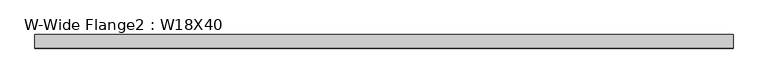
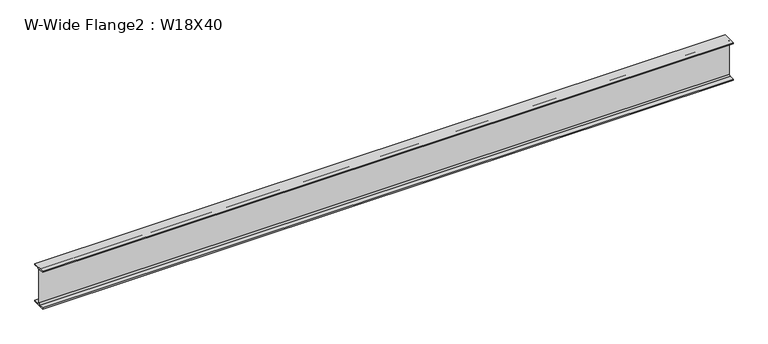
"""IFC4 building model written with IfcOpenShell, lengths in millimetres: beam geometry, W-Wide Flange2 : W18X40."""

from ifc_helpers import new_model, si_unit, point, frame, frame_2d, origin, place, context, project, spatial, polyline, circle_curve, trimmed, segment, composite_curve, outline, extrude, source, transform, mapped, element, save


def w_wide_flange2_w18x40_35908a48(model_context):
    return source(origin(), model_context, "Body", "SweptSolid", [
        extrude(outline(composite_curve([segment(polyline([(76.454, -213.995), (76.454, -227.33), (-76.454, -227.33), (-76.454, -213.995), (-20.828, -213.995)]), True, "CONTINUOUS"), segment(trimmed(circle_curve(frame_2d((-20.828, -197.1675)), 16.8275), [point((-20.828, -213.995))], [point((-4.0005, -197.1675))], True, "CARTESIAN"), True, "CONTINUOUS"), segment(polyline([(-4.0005, -197.1675), (-4.0005, 197.1675)]), True, "CONTINUOUS"), segment(trimmed(circle_curve(frame_2d((-20.828, 197.1675)), 16.8275), [point((-4.0005, 197.1675))], [point((-20.828, 213.995))], True, "CARTESIAN"), True, "CONTINUOUS"), segment(polyline([(-20.828, 213.995), (-76.454, 213.995), (-76.454, 227.33), (76.454, 227.33), (76.454, 213.995), (20.828, 213.995)]), True, "CONTINUOUS"), segment(trimmed(circle_curve(frame_2d((20.828, 197.1675)), 16.8275), [point((20.828, 213.995))], [point((4.0005, 197.1675))], True, "CARTESIAN"), True, "CONTINUOUS"), segment(polyline([(4.0005, 197.1675), (4.0005, -197.1675)]), True, "CONTINUOUS"), segment(trimmed(circle_curve(frame_2d((20.828, -197.1675)), 16.8275), [point((4.0005, -197.1675))], [point((20.828, -213.995))], True, "CARTESIAN"), True, "CONTINUOUS"), segment(polyline([(20.828, -213.995), (76.454, -213.995)]), True, "CONTINUOUS")], self_intersect=False)), frame((-3899.69375, 0.0, 0.0), z_axis=(1.0, 0.0, 0.0), x_axis=(0.0, 1.0, 0.0)), (0.0, 0.0, 1.0), 7856.5375),
    ])


if __name__ == "__main__":
    model = new_model("IFC4")
    model_context = context("Model", 3, world=origin())
    ifc_project = project(units=[si_unit("LENGTHUNIT", "METRE", prefix="MILLI")], contexts=[model_context])
    site = spatial("IfcSite", under=ifc_project)
    building = spatial("IfcBuilding", under=site)
    placement = place(None, origin())
    w_wide_flange2_w18x40_shape = w_wide_flange2_w18x40_35908a48(model_context)
    element("IfcBeam", 1, ObjectType="W-Wide Flange2 : W18X40", at=placement, inside=building, context=model_context, shape_type="MappedRepresentation", body=[
        mapped(w_wide_flange2_w18x40_shape, transform((0.0, 0.0, 0.0), x_axis=(1.0, 0.0, 0.0), y_axis=(0.0, 1.0, 0.0), z_axis=(0.0, 0.0, 1.0))),
    ])
    save(model, "model.ifc")

# Revit data of these elements
# Type "W-Wide Flange2 : W18X40"
#   Assembly Code = "B10"
#   W = 40
#   Length [instance default] = 5' - 0"
#   bf = 0' - 6.02"
#   d = 1' - 5.9"
#   k = 0' - 1 3/16"
#   k2 = 0' - 0.6625"
#   tf = 0' - 0.525"
#   tw = 0' - 0.315"
#   A = 0.0819444 SF
#   Structural Material [instance default] = Steel ASTM A992
# Element 1 (IfcBeam, "W-Wide Flange2 : W18X40")
#   Materials on its faces: "Steel ASTM A992"
# Materials
#   "Steel ASTM A992": class "Metal", colour RGB 199 199 199, transparency 0, Description = "Structural steel 50ksi", Cost = 0
